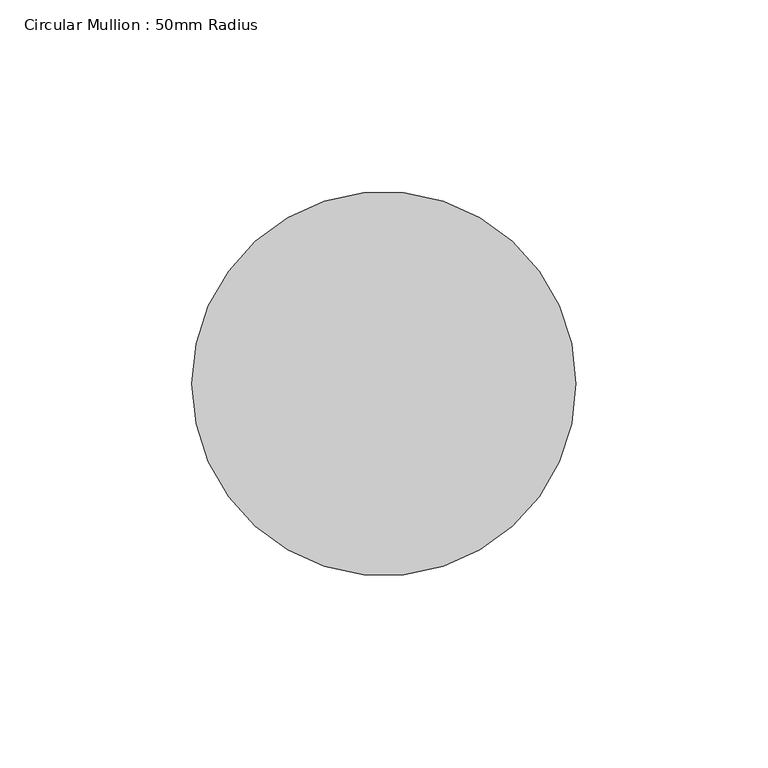
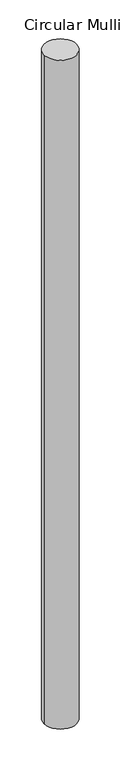
"""IFC4 building model written with IfcOpenShell, lengths in millimetres: member geometry, Circular Mullion : 50mm Radius."""

from ifc_helpers import new_model, si_unit, point, frame, frame_2d, origin, place, context, project, spatial, circle_curve, trimmed, segment, composite_curve, outline, extrude, source, transform, mapped, element, save


def circular_mullion_50mm_radius_14603ba2(model_context):
    return source(origin(), model_context, "Body", "SweptSolid", [
        extrude(outline(composite_curve([segment(trimmed(circle_curve(frame_2d((-50.0, 0.0)), 50.0), [point((0.0, 0.0))], [point((-100.0, 0.0))], False, "CARTESIAN"), True, "CONTINUOUS"), segment(trimmed(circle_curve(frame_2d((-50.0, 0.0)), 50.0), [point((-100.0, 0.0))], [point((0.0, 0.0))], False, "CARTESIAN"), True, "CONTINUOUS")], self_intersect=False)), frame((0.0, 0.0, -2172.055748), z_axis=(0.0, 0.0, 1.0), x_axis=(1.0, 0.0, 0.0)), (0.0, 0.0, 1.0), 2172.055748),
    ])


if __name__ == "__main__":
    model = new_model("IFC4")
    model_context = context("Model", 3, world=origin())
    ifc_project = project(units=[si_unit("LENGTHUNIT", "METRE", prefix="MILLI")], contexts=[model_context])
    site = spatial("IfcSite", under=ifc_project)
    building = spatial("IfcBuilding", under=site)
    placement = place(None, origin())
    circular_mullion_50mm_radius_shape = circular_mullion_50mm_radius_14603ba2(model_context)
    element("IfcMember", 1, ObjectType="Circular Mullion : 50mm Radius", at=placement, inside=building, context=model_context, shape_type="MappedRepresentation", body=[
        mapped(circular_mullion_50mm_radius_shape, transform((0.0, 0.0, 0.0), x_axis=(1.0, 0.0, 0.0), y_axis=(0.0, 1.0, 0.0), z_axis=(0.0, 0.0, 1.0))),
    ])
    save(model, "model.ifc")

# Revit data of these elements
# Type "Circular Mullion : 50mm Radius"
#   built-in parameter 1007350 = 0.164042 (stored number, unit not read)
# Element 1 (IfcMember, "Circular Mullion : 50mm Radius")
#   Materials on its faces: "Aluminium"
# Materials
#   "Aluminium": class "Metal", colour RGB 247 247 247, transparency 0, Description = "Aluminium 6061", Cost = 0
